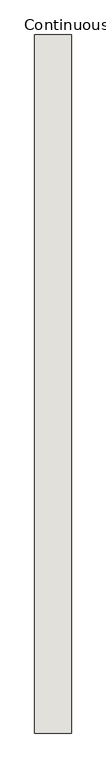
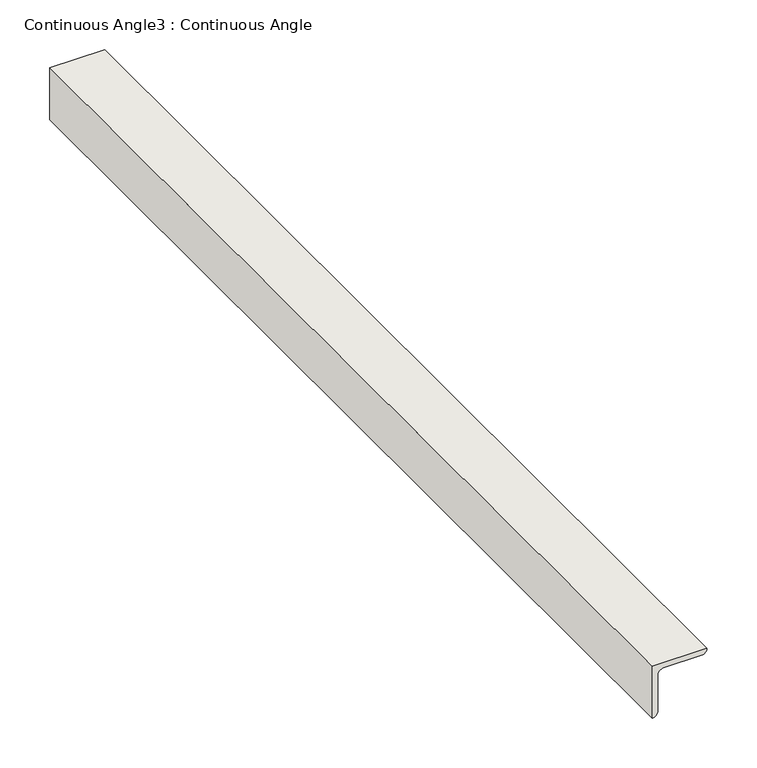
"""IFC4 building model written with IfcOpenShell, lengths in millimetres: wall geometry, Continuous Angle3 : Continuous Angle."""

from ifc_helpers import new_model, si_unit, point, frame, frame_2d, origin, place, context, project, spatial, polyline, circle_curve, trimmed, segment, composite_curve, outline, extrude, source, transform, mapped, element, save


def continuous_angle3_continuous_angle_3c84b8f5(model_context):
    return source(origin(), model_context, "Body", "SweptSolid", [
        extrude(outline(composite_curve([segment(polyline([(2260.6, 428979.0125), (2197.1, 428979.0125)]), True, "CONTINUOUS"), segment(trimmed(circle_curve(frame_2d((2203.45, 428979.0125)), 6.35), [point((2197.1, 428979.0125))], [point((2203.45, 428985.3625))], False, "CARTESIAN"), True, "CONTINUOUS"), segment(polyline([(2203.45, 428985.3625), (2247.9, 428985.3625)]), True, "CONTINUOUS"), segment(trimmed(circle_curve(frame_2d((2247.9, 428991.7125)), 6.35), [point((2247.9, 428985.3625))], [point((2254.25, 428991.7125))], True, "CARTESIAN"), True, "CONTINUOUS"), segment(polyline([(2254.25, 428991.7125), (2254.25, 429036.1625)]), True, "CONTINUOUS"), segment(trimmed(circle_curve(frame_2d((2260.6, 429036.1625)), 6.35), [point((2254.25, 429036.1625))], [point((2260.6, 429042.5125))], False, "CARTESIAN"), True, "CONTINUOUS"), segment(polyline([(2260.6, 429042.5125), (2260.6, 428979.0125)]), True, "CONTINUOUS")], self_intersect=False)), frame((0.0, 304.8, 0.0), z_axis=(0.0, 1.0, 0.0), x_axis=(0.0, 0.0, 1.0)), (0.0, 0.0, 1.0), 1209.675),
    ])


if __name__ == "__main__":
    model = new_model("IFC4")
    model_context = context("Model", 3, world=origin())
    ifc_project = project(units=[si_unit("LENGTHUNIT", "METRE", prefix="MILLI")], contexts=[model_context])
    site = spatial("IfcSite", under=ifc_project)
    building = spatial("IfcBuilding", under=site)
    placement = place(None, origin())
    continuous_angle3_continuous_angle_shape = continuous_angle3_continuous_angle_3c84b8f5(model_context)
    element("IfcWall", 1, ObjectType="Continuous Angle3 : Continuous Angle", at=placement, inside=building, context=model_context, shape_type="MappedRepresentation", body=[
        mapped(continuous_angle3_continuous_angle_shape, transform((0.0, 0.0, 0.0), x_axis=(1.0, 0.0, 0.0), y_axis=(0.0, 1.0, 0.0), z_axis=(0.0, 0.0, 1.0))),
    ])
    save(model, "model.ifc")

# Revit data of these elements
# Element 1 (IfcWall, "Continuous Angle3 : Continuous Angle")
#   Materials on its faces: "3\" X 3\" X 8\" L. CLIP ANGLES @ 4'-0\" O.C. MECH. FASTENED TO UNDERSIDE OF STRUCTURE OR SLAB - BOTH SIDES OF WALL"
# Materials
#   "3\" X 3\" X 8\" L. CLIP ANGLES @ 4'-0\" O.C. MECH. FASTENED TO UNDERSIDE OF STRUCTURE OR SLAB - BOTH SIDES OF WALL": class "Unassigned", colour RGB 210 209 208, transparency 0, Keynote = "M05121300.02", Cost = 0
